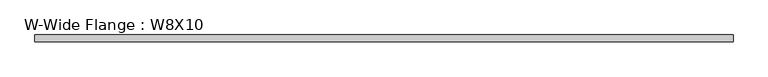
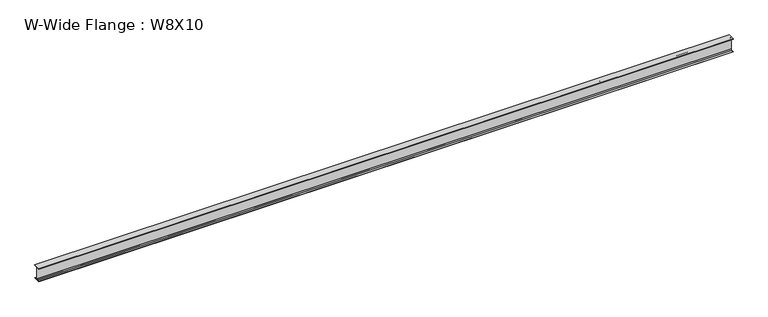
"""IFC4 building model written with IfcOpenShell, lengths in millimetres: beam geometry, W-Wide Flange : W8X10."""

from ifc_helpers import new_model, si_unit, point, frame, frame_2d, origin, place, context, project, spatial, polyline, circle_curve, trimmed, segment, composite_curve, outline, extrude, source, transform, mapped, element, save


def w_wide_flange_w8x10_852bdd75(model_context):
    return source(origin(), model_context, "Body", "SweptSolid", [
        extrude(outline(composite_curve([segment(polyline([(50.038, -94.996), (50.038, -100.203), (-50.038, -100.203), (-50.038, -94.996), (-14.4145, -94.996)]), True, "CONTINUOUS"), segment(trimmed(circle_curve(frame_2d((-14.4145, -82.7405)), 12.2555), [point((-14.4145, -94.996))], [point((-2.159, -82.7405))], True, "CARTESIAN"), True, "CONTINUOUS"), segment(polyline([(-2.159, -82.7405), (-2.159, 82.7405)]), True, "CONTINUOUS"), segment(trimmed(circle_curve(frame_2d((-14.4145, 82.7405)), 12.2555), [point((-2.159, 82.7405))], [point((-14.4145, 94.996))], True, "CARTESIAN"), True, "CONTINUOUS"), segment(polyline([(-14.4145, 94.996), (-50.038, 94.996), (-50.038, 100.203), (50.038, 100.203), (50.038, 94.996), (14.4145, 94.996)]), True, "CONTINUOUS"), segment(trimmed(circle_curve(frame_2d((14.4145, 82.7405)), 12.2555), [point((14.4145, 94.996))], [point((2.159, 82.7405))], True, "CARTESIAN"), True, "CONTINUOUS"), segment(polyline([(2.159, 82.7405), (2.159, -82.7405)]), True, "CONTINUOUS"), segment(trimmed(circle_curve(frame_2d((14.4145, -82.7405)), 12.2555), [point((2.159, -82.7405))], [point((14.4145, -94.996))], True, "CARTESIAN"), True, "CONTINUOUS"), segment(polyline([(14.4145, -94.996), (50.038, -94.996)]), True, "CONTINUOUS")], self_intersect=False)), frame((-5037.6903421, 0.0, 0.0), z_axis=(1.0, 0.0, 0.0), x_axis=(0.0, 1.0, 0.0)), (0.0, 0.0, 1.0), 10075.3806843),
    ])


if __name__ == "__main__":
    model = new_model("IFC4")
    model_context = context("Model", 3, world=origin())
    ifc_project = project(units=[si_unit("LENGTHUNIT", "METRE", prefix="MILLI")], contexts=[model_context])
    site = spatial("IfcSite", under=ifc_project)
    building = spatial("IfcBuilding", under=site)
    placement = place(None, origin())
    w_wide_flange_w8x10_shape = w_wide_flange_w8x10_852bdd75(model_context)
    element("IfcBeam", 1, ObjectType="W-Wide Flange : W8X10", at=placement, inside=building, context=model_context, shape_type="MappedRepresentation", body=[
        mapped(w_wide_flange_w8x10_shape, transform((0.0, 0.0, 0.0), x_axis=(1.0, 0.0, 0.0), y_axis=(0.0, 1.0, 0.0), z_axis=(0.0, 0.0, 1.0))),
    ])
    save(model, "model.ifc")

# Revit data of these elements
# Type "W-Wide Flange : W8X10"
#   Assembly Code = "B10"
#   W = 10
#   Length [instance default] = 5' - 0"
#   bf = 0' - 3.94"
#   d = 0' - 7.89"
#   k = 0' - 0 11/16"
#   k2 = 0' - 0.4825"
#   tf = 0' - 0.205"
#   tw = 0' - 0.17"
#   A = 0.0205556 SF
#   Structural Material [instance default] = Steel ASTM A992
# Element 1 (IfcBeam, "W-Wide Flange : W8X10")
#   Structural Material = none
# Materials
#   "Steel ASTM A992": class "Metal", colour RGB 189 187 185, transparency 0, Description = "Structural steel 50ksi", Cost = 0
